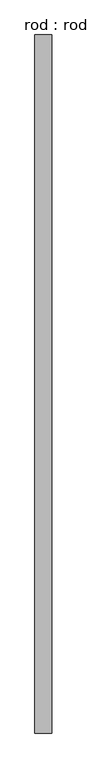
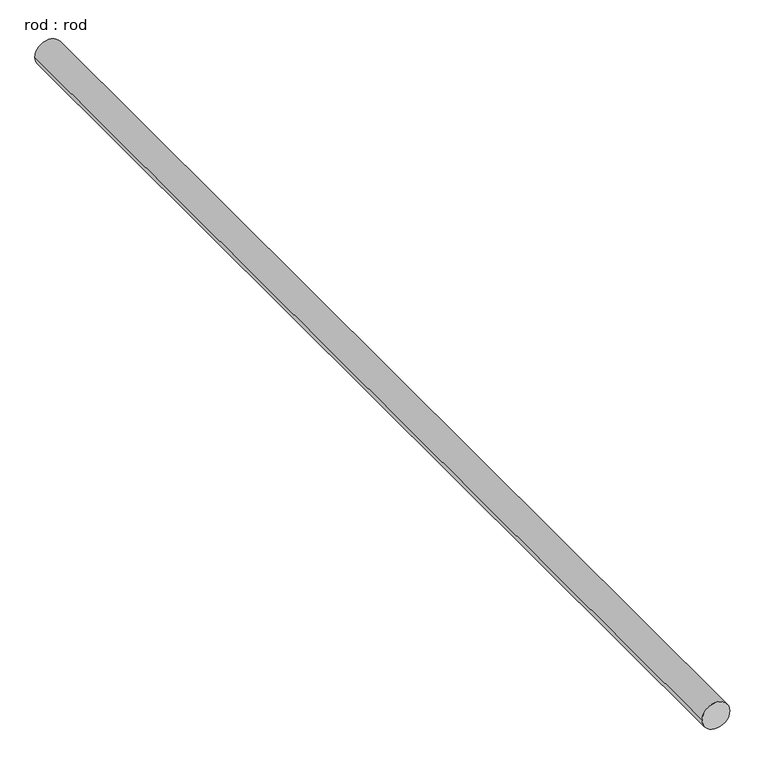
"""IFC4 building model written with IfcOpenShell, lengths in millimetres: proxy geometry, rod : rod."""

import ifcopenshell
import ifcopenshell.guid

model = None  # the IFC model being written
_history = None  # IfcOwnerHistory: only IFC2X3 demands one
_inside = {}  # id of a spatial element -> (the spatial element, [elements in it])
_under = {}  # id of a project, library or spatial element -> (it, [spatial elements below it])
_declared = {}  # id of a project -> (the project, [libraries it declares])
_typed = {}  # id of a type object -> (the type object, [elements of that type])
_made_of = {}  # id of a material, layer set ... -> (it, [elements and type objects made of it])


def new_model(schema):
    """Start an empty IFC model of exactly this schema.

    Asked for "IFC4X3", IfcOpenShell would pick the latest addendum, in which some entities
    have other attributes; the version numbers below select the first issue.
    IFC2X3 requires an IfcOwnerHistory on every rooted entity: one is made here for all.
    """
    global model, _history
    if schema == "IFC4X3":
        model = ifcopenshell.file(schema_version=(4, 3, 0, 0))
    else:
        model = ifcopenshell.file(schema=schema)
    _inside.clear()
    _under.clear()
    _declared.clear()
    _typed.clear()
    _made_of.clear()
    _history = None
    if model.schema == "IFC2X3":
        org = make("IfcOrganization", Name="unknown")
        user = make(
            "IfcPersonAndOrganization",
            ThePerson=make("IfcPerson", FamilyName="unknown"),
            TheOrganization=org,
        )
        app = make(
            "IfcApplication",
            ApplicationDeveloper=org,
            Version="unknown",
            ApplicationFullName="unknown",
            ApplicationIdentifier="unknown",
        )
        _history = make(
            "IfcOwnerHistory",
            OwningUser=user,
            OwningApplication=app,
            ChangeAction="ADDED",
            CreationDate=0,
        )
    return model


def make(cls, **values):
    """One entity of the class cls with the attributes given. An attribute that is None is left unset."""
    return model.create_entity(
        cls, **{name: value for name, value in values.items() if value is not None}
    )


def rooted(cls, **values):
    """An entity with a GlobalId (a new one), such as an element, a storey or a relation."""
    return make(cls, GlobalId=ifcopenshell.guid.new(), OwnerHistory=_history, **values)


def si_unit(unit_type, name, prefix=None):
    """IfcSIUnit, for example si_unit("LENGTHUNIT", "METRE", prefix="MILLI")."""
    return make("IfcSIUnit", UnitType=unit_type, Prefix=prefix, Name=name)


def assignment(units):
    """IfcUnitAssignment: the units of a project."""
    return None if units is None else make("IfcUnitAssignment", Units=units)


def point(xyz):
    """IfcCartesianPoint."""
    return None if xyz is None else make("IfcCartesianPoint", Coordinates=xyz)


def direction(xyz):
    """IfcDirection."""
    return None if xyz is None else make("IfcDirection", DirectionRatios=xyz)


def frame(location, z_axis=None, x_axis=None):
    """IfcAxis2Placement3D, a coordinate frame: its origin and axes. An axis left out is left unset."""
    return make(
        "IfcAxis2Placement3D",
        Location=point(location),
        Axis=direction(z_axis),
        RefDirection=direction(x_axis),
    )


def frame_2d(location, x_axis=None):
    """IfcAxis2Placement2D, a coordinate frame in the plane: its origin and x axis."""
    return make(
        "IfcAxis2Placement2D", Location=point(location), RefDirection=direction(x_axis)
    )


def origin():
    """The frame at (0, 0, 0) with its axes left unset."""
    return frame((0.0, 0.0, 0.0))


def place(relative_to, where):
    """IfcLocalPlacement: puts the frame where relative to a parent placement (None: the world)."""
    return make(
        "IfcLocalPlacement", PlacementRelTo=relative_to, RelativePlacement=where
    )


def context(
    kind, dimensions, precision=None, world=None, true_north=None, identifier=None
):
    """IfcGeometricRepresentationContext, for example the 3D "Model" context."""
    return make(
        "IfcGeometricRepresentationContext",
        ContextIdentifier=identifier,
        ContextType=kind,
        CoordinateSpaceDimension=dimensions,
        Precision=precision,
        WorldCoordinateSystem=world,
        TrueNorth=true_north,
    )


def project(units=None, contexts=None):
    """IfcProject with its units and contexts."""
    return rooted(
        "IfcProject",
        Name="project",
        RepresentationContexts=contexts,
        UnitsInContext=assignment(units),
    )


def spatial(cls, under=None, at=None, **own):
    """A site, building, storey or space (cls), placed at a placement, below another one or the project."""
    s = rooted(cls, ObjectPlacement=at, **own)
    if under is not None:
        _under.setdefault(under.id(), (under, []))[1].append(s)
    return s


def circle_curve(where, radius):
    """IfcCircle in the frame where."""
    return make("IfcCircle", Position=where, Radius=radius)


def trimmed(basis, trim1, trim2, sense, master):
    """IfcTrimmedCurve: the piece of a basis curve between two trims."""
    return make(
        "IfcTrimmedCurve",
        BasisCurve=basis,
        Trim1=trim1,
        Trim2=trim2,
        SenseAgreement=sense,
        MasterRepresentation=master,
    )


def segment(curve, same_sense, transition):
    """IfcCompositeCurveSegment."""
    return make(
        "IfcCompositeCurveSegment",
        Transition=transition,
        SameSense=same_sense,
        ParentCurve=curve,
    )


def composite_curve(segments, self_intersect=None):
    """IfcCompositeCurve: segments joined end to end."""
    return make("IfcCompositeCurve", Segments=segments, SelfIntersect=self_intersect)


def outline(outer, holes=None, kind="AREA"):
    """IfcArbitraryClosedProfileDef: a profile drawn as a closed curve; with holes, ...WithVoids."""
    if holes is None:
        return make("IfcArbitraryClosedProfileDef", ProfileType=kind, OuterCurve=outer)
    return make(
        "IfcArbitraryProfileDefWithVoids",
        ProfileType=kind,
        OuterCurve=outer,
        InnerCurves=holes,
    )


def extrude(swept, where, along, depth):
    """IfcExtrudedAreaSolid: the profile swept, set in the frame where, extruded along a direction by depth."""
    return make(
        "IfcExtrudedAreaSolid",
        SweptArea=swept,
        Position=where,
        ExtrudedDirection=direction(along),
        Depth=depth,
    )


def shape(context_of_items, identifier, shape_type, items):
    """IfcShapeRepresentation: the items that make up one representation, for example the "Body"."""
    return make(
        "IfcShapeRepresentation",
        ContextOfItems=context_of_items,
        RepresentationIdentifier=identifier,
        RepresentationType=shape_type,
        Items=items,
    )


def source(mapping_origin, context_of_items, identifier, shape_type, items):
    """IfcRepresentationMap: a shape defined once, which mapped items show again and again."""
    return make(
        "IfcRepresentationMap",
        MappingOrigin=mapping_origin,
        MappedRepresentation=shape(context_of_items, identifier, shape_type, items),
    )


def transform(
    local_origin,
    x_axis=None,
    y_axis=None,
    z_axis=None,
    scale=None,
    scale2=None,
    scale3=None,
    uniform=True,
):
    """IfcCartesianTransformationOperator3D, or its non-uniform kind. x_axis, y_axis, z_axis: its Axis1, 2, 3."""
    if uniform:
        return make(
            "IfcCartesianTransformationOperator3D",
            Axis1=direction(x_axis),
            Axis2=direction(y_axis),
            LocalOrigin=point(local_origin),
            Scale=scale,
            Axis3=direction(z_axis),
        )
    return make(
        "IfcCartesianTransformationOperator3DnonUniform",
        Axis1=direction(x_axis),
        Axis2=direction(y_axis),
        LocalOrigin=point(local_origin),
        Scale=scale,
        Axis3=direction(z_axis),
        Scale2=scale2,
        Scale3=scale3,
    )


def mapped(mapping_source, mapping_target):
    """IfcMappedItem: shows the shape of a source again, moved by a transform."""
    return make(
        "IfcMappedItem", MappingSource=mapping_source, MappingTarget=mapping_target
    )


def made_of(thing, what):
    """Note that an element or type object is made of a material, layer set ...; save() writes the relation."""
    if what is not None:
        _made_of.setdefault(what.id(), (what, []))[1].append(thing)
    return thing


def element(
    cls,
    number,
    at=None,
    inside=None,
    cuts=None,
    type_object=None,
    material=None,
    context=None,
    identifier="Body",
    shape_type=None,
    held_by="IfcProductDefinitionShape",
    body=None,
    shapes=None,
    **own,
):
    """One element of the class cls, such as IfcWall. Its Tag is "e" and its number.

    at: its placement. inside: the storey or other place that contains it. cuts: it is an
    opening in that element (IfcRelVoidsElement). A single representation is given by context,
    identifier, shape_type and body (its items); several are given by shapes. held_by: the class
    of the entity that holds the representations. save() writes the other relations.
    """
    e = rooted(cls, Tag="e%d" % number, ObjectPlacement=at, **own)
    if body is not None:
        shapes = [shape(context, identifier, shape_type, body)]
    if shapes is not None:
        e.Representation = make(held_by, Representations=shapes)
    if inside is not None:
        _inside.setdefault(inside.id(), (inside, []))[1].append(e)
    if cuts is not None:
        rooted(
            "IfcRelVoidsElement", RelatingBuildingElement=cuts, RelatedOpeningElement=e
        )
    if type_object is not None:
        _typed.setdefault(type_object.id(), (type_object, []))[1].append(e)
    return made_of(e, material)


def aggregate(whole, parts):
    """IfcRelAggregates: a whole, such as a stair, and the parts it consists of."""
    return rooted("IfcRelAggregates", RelatingObject=whole, RelatedObjects=parts)


def save(model, path):
    """Write the relations noted so far, then the file.

    IfcRelAggregates (storeys below a building ...), IfcRelContainedInSpatialStructure (elements
    in a storey), IfcRelDefinesByType, IfcRelAssociatesMaterial and IfcRelDeclares: one each for
    every whole, place, type object, material and project.
    """
    for whole, parts in _under.values():
        aggregate(whole, parts)
    for where, things in _inside.values():
        rooted(
            "IfcRelContainedInSpatialStructure",
            RelatedElements=things,
            RelatingStructure=where,
        )
    for kind, things in _typed.values():
        rooted("IfcRelDefinesByType", RelatedObjects=things, RelatingType=kind)
    for what, things in _made_of.values():
        rooted("IfcRelAssociatesMaterial", RelatedObjects=things, RelatingMaterial=what)
    for by, libraries in _declared.values():
        rooted("IfcRelDeclares", RelatingContext=by, RelatedDefinitions=libraries)
    model.write(path)


def rod_rod_a851ec8b(model_context):
    return source(origin(), model_context, "Body", "SweptSolid", [
        extrude(outline(composite_curve([segment(trimmed(circle_curve(frame_2d((0.0108462, 0.0)), 200.0), [point((0.0108462, 200.0))], [point((0.0108462, -200.0))], False, "CARTESIAN"), True, "CONTINUOUS"), segment(trimmed(circle_curve(frame_2d((0.0108462, 0.0)), 200.0), [point((0.0108462, -200.0))], [point((0.0108462, 200.0))], False, "CARTESIAN"), True, "CONTINUOUS")], self_intersect=False)), frame((0.0, -4268.3824958, 0.0), z_axis=(0.0, 1.0, 0.0), x_axis=(0.0, 0.0, 1.0)), (0.0, 0.0, 1.0), 16722.2222222),
    ])


if __name__ == "__main__":
    model = new_model("IFC4")
    model_context = context("Model", 3, world=origin())
    ifc_project = project(units=[si_unit("LENGTHUNIT", "METRE", prefix="MILLI")], contexts=[model_context])
    site = spatial("IfcSite", under=ifc_project)
    building = spatial("IfcBuilding", under=site)
    placement = place(None, origin())
    rod_rod_shape = rod_rod_a851ec8b(model_context)
    element("IfcBuildingElementProxy", 1, Name="rod : rod", ObjectType="rod : rod", at=placement, inside=building, context=model_context, shape_type="MappedRepresentation", body=[
        mapped(rod_rod_shape, transform((0.0, 0.0, 0.0), x_axis=(1.0, 0.0, 0.0), y_axis=(0.0, 1.0, 0.0), z_axis=(0.0, 0.0, 1.0))),
    ])
    save(model, "model.ifc")

# Revit data of these elements
# Type "rod : rod"
#   Default Elevation = 0
